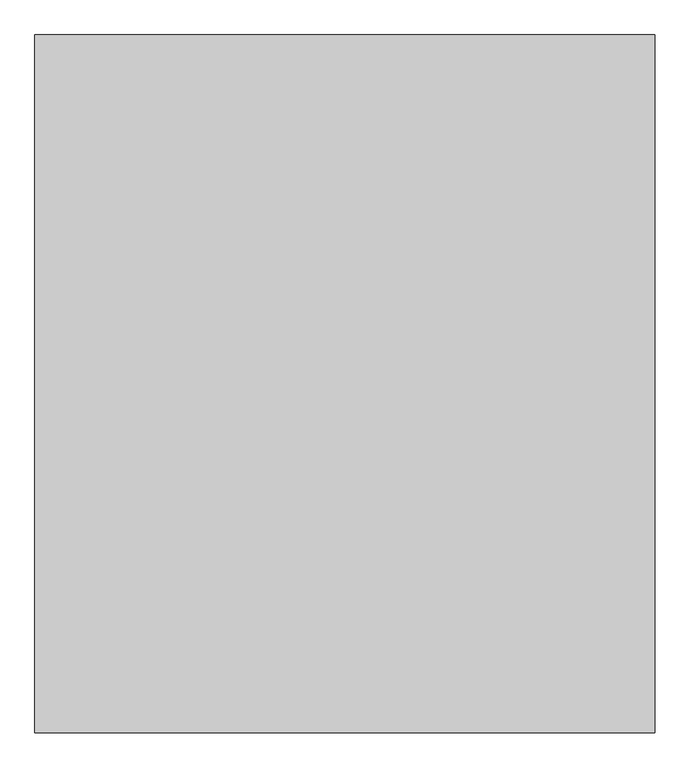
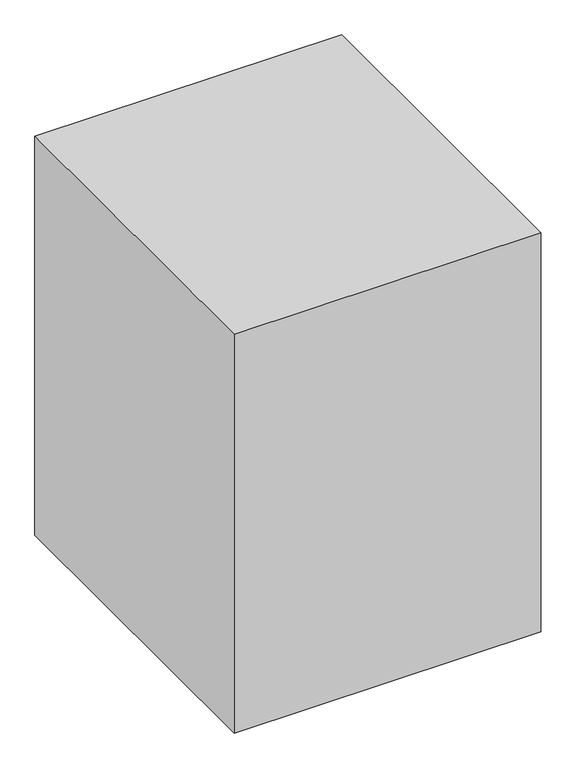
"""IFC4 building model written with IfcOpenShell, lengths in millimetres: proxy geometry, Space Planning Box_hec : Space Planning Box_hec."""

from ifc_helpers import new_model, si_unit, origin, origin_with_axes, place, context, project, spatial, polyline, outline, extrude, source, transform, mapped, element, save


def generic_models_971c0b89(model_context):
    return source(origin(), model_context, "Body", "SweptSolid", [
        extrude(outline(polyline([(2000.0, 2250.0), (2000.0, -2250.0), (-2000.0, -2250.0), (-2000.0, 2250.0), (2000.0, 2250.0)])), origin_with_axes(), (0.0, 0.0, 1.0), 5500.0),
    ])


if __name__ == "__main__":
    model = new_model("IFC4")
    model_context = context("Model", 3, world=origin())
    ifc_project = project(units=[si_unit("LENGTHUNIT", "METRE", prefix="MILLI")], contexts=[model_context])
    site = spatial("IfcSite", under=ifc_project)
    building = spatial("IfcBuilding", under=site)
    placement = place(None, origin())
    generic_models_shape = generic_models_971c0b89(model_context)
    element("IfcBuildingElementProxy", 1, Name="Space Planning Box_hec : Space Planning Box_hec", ObjectType="Space Planning Box_hec : Space Planning Box_hec", at=placement, inside=building, context=model_context, shape_type="MappedRepresentation", body=[
        mapped(generic_models_shape, transform((0.0, 0.0, 0.0), x_axis=(1.0, 0.0, 0.0), y_axis=(0.0, 1.0, 0.0), z_axis=(0.0, 0.0, 1.0))),
    ])
    save(model, "model.ifc")

# Revit data of these elements
# Type "Space Planning Box_hec : Space Planning Box_hec"
#   Type Comments = "..."
#   Room Name [instance default] = "?"
#   Interior Finish [instance default] = ""
#   Exterior Finish [instance default] = ""
#   Department [instance default] = ""
#   Assembly Code = "..."
#   ceiling height [instance default] = 0
#   Width [instance default] = 1524 mm
#   Program Area [instance default] = 0.00 m²
#   Length [instance default] = 1524 mm
#   Height [instance default] = 1524 mm
#   Area [instance default] = 2.32258 m²
#   Fill Color [instance default] = Cyan
#   Default Elevation = 0
# Element 1 (IfcBuildingElementProxy, "Space Planning Box_hec : Space Planning Box_hec")
#   Room Name = "Toilet (M)"
#   Exterior Finish = "N/A..N/A,,EW2..N/A..N/A"
#   Department = "AR"
#   Width = 4000 mm
#   Program Area = 18.00 m²
#   Length = 4500 mm
#   Height = 5500 mm
#   Area = 18.00 m²
#   Materials on its faces: "Cyan"
# Materials
#   "Cyan": class "Generic", colour RGB 0 255 255, transparency 0.2, Cost = 0
